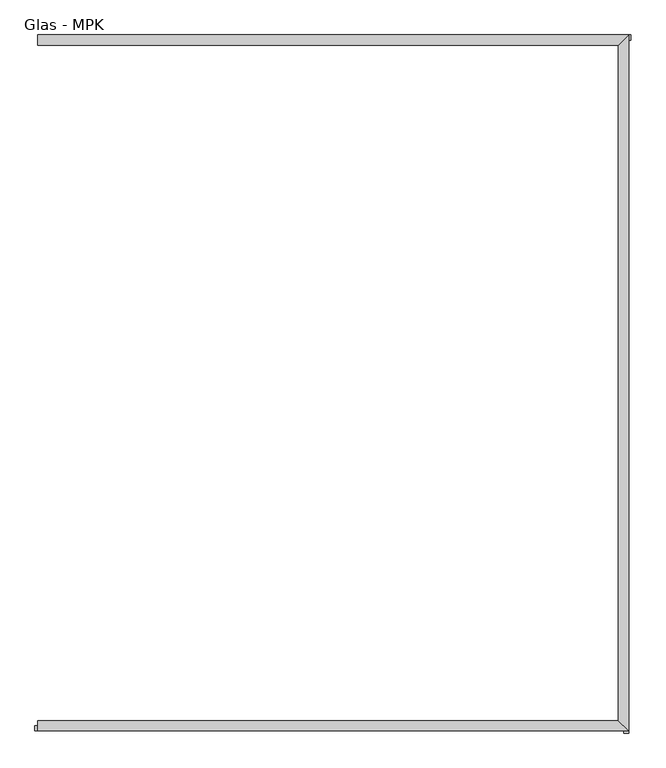
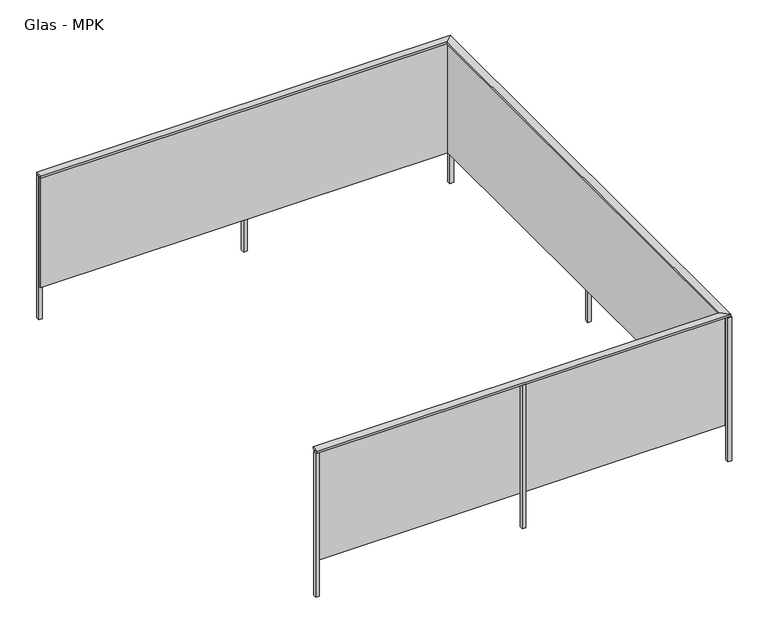
"""IFC4 building model written with IfcOpenShell, lengths in millimetres: railing geometry, Glas - MPK."""

from ifc_helpers import new_model, si_unit, frame, origin, place, context, project, spatial, polyline, outline, extrude, faceted_brep, source, transform, mapped, element, save


def glas_mpk_b2065e46(model_context):
    return source(origin(), model_context, "Body", "SolidModel", [
        faceted_brep([(28810.8437289, 1294.9571597, 6843.2628643), (28810.8437289, 1244.9571597, 6843.2628643), (28810.8437289, 1244.9571597, 6856.7371357), (28810.8437289, 1294.9571597, 6856.7371357), (31650.8437289, 1294.9571597, 6843.2628643), (31600.8437289, 1244.9571597, 6843.2628643), (31600.8437289, 1244.9571597, 6856.7371357), (31650.8437289, 1294.9571597, 6856.7371357), (31650.8437289, -2045.7721864, 6843.2628643), (31600.8437289, -1995.7721864, 6843.2628643), (31600.8437289, -1995.7721864, 6856.7371357), (31650.8437289, -2045.7721864, 6856.7371357), (28810.8437289, -2045.7721864, 6843.2628643), (28810.8437289, -2045.7721864, 6856.7371357), (28810.8437289, -1995.7721864, 6856.7371357), (28810.8437289, -1995.7721864, 6843.2628643)], [[[0, 1, 2, 3]], [[1, 0, 4, 5]], [[2, 1, 5, 6]], [[3, 2, 6, 7]], [[0, 3, 7, 4]], [[5, 4, 8, 9]], [[6, 5, 9, 10]], [[7, 6, 10, 11]], [[4, 7, 11, 8]], [[12, 13, 14, 15]], [[9, 8, 12, 15]], [[10, 9, 15, 14]], [[11, 10, 14, 13]], [[8, 11, 13, 12]]]),
        faceted_brep([(28810.8437289, 1254.9571597, 6842.8769824), (28810.8437289, 1269.1492837, 6842.8769824), (28810.8437289, 1269.1492837, 6042.8769824), (28810.8437289, 1254.9571597, 6042.8769824), (31610.8437289, 1254.9571597, 6842.8769824), (31625.0358529, 1269.1492837, 6842.8769824), (31625.0358529, 1269.1492837, 6042.8769824), (31610.8437289, 1254.9571597, 6042.8769824), (31610.8437289, -2005.7721864, 6842.8769824), (31625.0358529, -2019.9643104, 6842.8769824), (31625.0358529, -2019.9643104, 6042.8769824), (31610.8437289, -2005.7721864, 6042.8769824), (28810.8437289, -2005.7721864, 6842.8769824), (28810.8437289, -2005.7721864, 6042.8769824), (28810.8437289, -2019.9643104, 6042.8769824), (28810.8437289, -2019.9643104, 6842.8769824)], [[[0, 1, 2, 3]], [[1, 0, 4, 5]], [[2, 1, 5, 6]], [[3, 2, 6, 7]], [[0, 3, 7, 4]], [[5, 4, 8, 9]], [[6, 5, 9, 10]], [[7, 6, 10, 11]], [[4, 7, 11, 8]], [[12, 13, 14, 15]], [[9, 8, 12, 15]], [[10, 9, 15, 14]], [[11, 10, 14, 13]], [[8, 11, 13, 12]]]),
        extrude(outline(polyline([(30242.0937289, -2020.7721864), (30242.0937289, -2045.7721864), (30217.0937289, -2045.7721864), (30217.0937289, -2020.7721864), (30242.0937289, -2020.7721864)])), frame((0.0, 0.0, 5800.0), z_axis=(0.0, 0.0, 1.0), x_axis=(1.0, 0.0, 0.0)), (0.0, 0.0, 1.0), 1043.2628643),
        extrude(outline(polyline([(31625.8437289, -362.9075133), (31650.8437289, -362.9075133), (31650.8437289, -387.9075133), (31625.8437289, -387.9075133), (31625.8437289, -362.9075133)])), frame((0.0, 0.0, 5800.0), z_axis=(0.0, 0.0, 1.0), x_axis=(1.0, 0.0, 0.0)), (0.0, 0.0, 1.0), 1043.2628643),
        extrude(outline(polyline([(30217.0937289, 1269.9571597), (30217.0937289, 1294.9571597), (30242.0937289, 1294.9571597), (30242.0937289, 1269.9571597), (30217.0937289, 1269.9571597)])), frame((0.0, 0.0, 5800.0), z_axis=(0.0, 0.0, 1.0), x_axis=(1.0, 0.0, 0.0)), (0.0, 0.0, 1.0), 1043.2628643),
        extrude(outline(polyline([(31625.8437289, -2030.7721864), (31650.8437289, -2030.7721864), (31650.8437289, -2055.7721864), (31625.8437289, -2055.7721864), (31625.8437289, -2030.7721864)])), frame((0.0, 0.0, 5800.0), z_axis=(0.0, 0.0, 1.0), x_axis=(1.0, 0.0, 0.0)), (0.0, 0.0, 1.0), 1043.2628643),
        extrude(outline(polyline([(31635.8437289, 1269.9571597), (31635.8437289, 1294.9571597), (31660.8437289, 1294.9571597), (31660.8437289, 1269.9571597), (31635.8437289, 1269.9571597)])), frame((0.0, 0.0, 5800.0), z_axis=(0.0, 0.0, 1.0), x_axis=(1.0, 0.0, 0.0)), (0.0, 0.0, 1.0), 1043.2628643),
        extrude(outline(polyline([(28823.3437289, -2020.7721864), (28823.3437289, -2045.7721864), (28798.3437289, -2045.7721864), (28798.3437289, -2020.7721864), (28823.3437289, -2020.7721864)])), frame((0.0, 0.0, 5800.0), z_axis=(0.0, 0.0, 1.0), x_axis=(1.0, 0.0, 0.0)), (0.0, 0.0, 1.0), 1043.2628643),
        extrude(outline(polyline([(28810.8437289, 1269.9571597), (28810.8437289, 1294.9571597), (28835.8437289, 1294.9571597), (28835.8437289, 1269.9571597), (28810.8437289, 1269.9571597)])), frame((0.0, 0.0, 5800.0), z_axis=(0.0, 0.0, 1.0), x_axis=(1.0, 0.0, 0.0)), (0.0, 0.0, 1.0), 1043.2628643),
    ])


if __name__ == "__main__":
    model = new_model("IFC4")
    model_context = context("Model", 3, world=origin())
    ifc_project = project(units=[si_unit("LENGTHUNIT", "METRE", prefix="MILLI")], contexts=[model_context])
    site = spatial("IfcSite", under=ifc_project)
    building = spatial("IfcBuilding", under=site)
    placement = place(None, origin())
    glas_mpk_shape = glas_mpk_b2065e46(model_context)
    element("IfcRailing", 1, ObjectType="Glas - MPK", at=placement, inside=building, context=model_context, shape_type="MappedRepresentation", body=[
        mapped(glas_mpk_shape, transform((0.0, 0.0, 0.0), x_axis=(1.0, 0.0, 0.0), y_axis=(0.0, 1.0, 0.0), z_axis=(0.0, 0.0, 1.0))),
    ])
    save(model, "model.ifc")

# Revit data of these elements
# Element 1 (IfcRailing, "Glas - MPK")
#   Materials on its faces: "Metal - Aluminum", "Window - Glass"
# Materials
#   "Metal - Aluminum": class "Unassigned", colour RGB 247 247 247, transparency 0, Comments = "Rendering appearance not upgraded "
#   "Window - Glass": class "Glas", colour RGB 128 128 255, transparency 0.75
